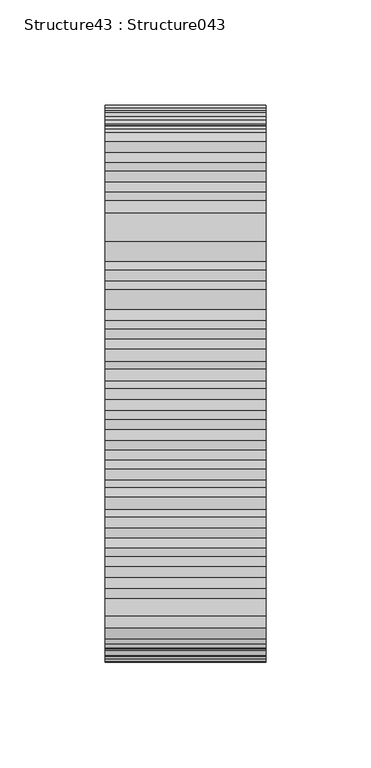
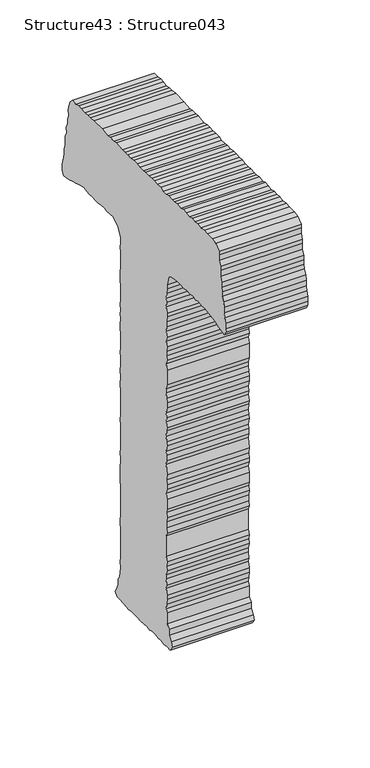
"""IFC4 building model written with IfcOpenShell, lengths in millimetres: proxy geometry, Structure43 : Structure043."""

from ifc_helpers import new_model, si_unit, frame, origin, place, context, project, spatial, polyline, outline, extrude, source, transform, mapped, element, save


def structure43_structure043_932cc00d(model_context):
    return source(origin(), model_context, "Body", "SweptSolid", [
        extrude(outline(polyline([(256415.821603, 3992.8375436), (256417.5818541, 3987.0048063), (256418.7644476, 3982.8793681), (256418.1627209, 3978.2035506), (256419.3437098, 3972.9372387), (256419.922972, 3969.418341), (256421.7056876, 3964.1343784), (256421.103961, 3959.4617701), (256423.4434743, 3954.7506513), (256423.4434743, 3951.2606365), (256423.4434743, 3945.9766739), (256425.2037254, 3940.718385), (256425.2037254, 3937.1930689), (256426.3638545, 3931.3346579), (256427.5448434, 3927.2332888), (256428.7258323, 3923.1319197), (256428.7258323, 3917.8479571), (256425.7845923, 3914.3499193), (256419.922972, 3914.9307861), (256415.2423407, 3916.0909152), (256411.1425762, 3917.8479571), (256406.4619449, 3918.4480792), (256402.9398381, 3919.6066036), (256394.1369778, 3921.9733953), (256388.8786889, 3921.3748778), (256384.7773198, 3920.7908018), (256380.074224, 3921.3748778), (256374.2366728, 3920.7908018), (256370.1353038, 3920.7908018), (256365.432208, 3921.9733953), (256360.173919, 3921.9733953), (256356.6518122, 3921.3748778), (256350.790192, 3921.9733953), (256346.1111652, 3921.9733953), (256337.9100317, 3916.6653636), (256333.7861981, 3909.0627475), (256334.3879248, 3904.3901392), (256334.967187, 3899.1061766), (256334.3879248, 3894.4030808), (256334.3879248, 3885.6210804), (256333.7861981, 3879.7610648), (256334.967187, 3875.0772243), (256334.967187, 3866.8776953), (256333.7861981, 3861.0192843), (256333.7861981, 3857.5019912), (256334.3879248, 3851.6612309), (256333.7861981, 3848.1166595), (256334.967187, 3842.8583706), (256333.7861981, 3837.6000817), (256334.967187, 3834.0474873), (256334.3879248, 3828.2163546), (256334.967187, 3823.5341187), (256334.967187, 3819.4150989), (256334.3879248, 3814.148787), (256334.3879248, 3800.6717138), (256334.967187, 3795.4037973), (256333.7861981, 3791.3056374), (256333.7861981, 3786.0280932), (256334.967187, 3776.6427615), (256333.7861981, 3773.11905), (256334.967187, 3763.759392), (256333.7861981, 3759.0595054), (256333.7861981, 3749.117376), (256334.3879248, 3744.4158848), (256333.7861981, 3738.5574738), (256334.3879248, 3735.0578314), (256334.967187, 3729.7738688), (256333.7861981, 3725.0996559), (256334.3879248, 3720.9726131), (256333.7861981, 3716.2887726), (256333.7861981, 3706.3289925), (256334.3879248, 3702.229228), (256334.967187, 3696.3884676), (256334.3879248, 3692.2710525), (256334.3879248, 3688.1873341), (256334.967187, 3683.4858429), (256334.967187, 3668.8261762), (256333.7861981, 3664.7440624), (256333.7861981, 3655.3587307), (256334.3879248, 3649.5003197), (256334.3879248, 3640.7167147), (256333.7861981, 3636.0408972), (256334.967187, 3631.3410106), (256334.967187, 3627.2396415), (256333.7861981, 3622.555801), (256334.3879248, 3617.2718384), (256334.3879248, 3612.5976255), (256333.7861981, 3607.8961343), (256334.3879248, 3602.6298224), (256334.3879248, 3594.4286888), (256334.967187, 3589.7544759), (256334.3879248, 3583.8864372), (256335.5464492, 3574.5107332), (256337.9100317, 3570.9854171), (256338.4892939, 3565.1254015), (256339.6702828, 3561.6257591), (256342.5890584, 3555.7416744), (256339.6702828, 3552.242032), (256334.967187, 3552.242032), (256330.2881603, 3551.6675836), (256324.4265401, 3551.0658569), (256320.9044332, 3551.0658569), (256316.2254065, 3551.6675836), (256306.843284, 3551.6675836), (256301.5833905, 3551.0658569), (256296.8802947, 3551.6675836), (256291.6204012, 3551.6675836), (256287.5206367, 3551.0658569), (256283.3968031, 3552.242032), (256278.7177764, 3552.242032), (256273.4354184, 3551.6675836), (256269.3565138, 3552.242032), (256264.6774871, 3551.0658569), (256258.7934024, 3552.242032), (256254.1127711, 3551.6675836), (256251.1715311, 3556.3417965), (256252.9317822, 3560.441561), (256255.8746268, 3565.1254015), (256255.8746268, 3570.9854171), (256258.7934024, 3574.5107332), (256259.3726646, 3585.0706354), (256260.5536535, 3588.5702778), (256259.9743913, 3593.2541183), (256259.3726646, 3598.5284533), (256259.3726646, 3602.6298224), (256260.5536535, 3608.4705827), (256259.9743913, 3612.0135494), (256260.5536535, 3617.8559144), (256260.5536535, 3621.9813526), (256259.3726646, 3626.6571701), (256259.9743913, 3630.7392839), (256259.3726646, 3635.4407751), (256260.5536535, 3640.114988), (256260.5536535, 3660.0682449), (256259.3726646, 3663.5598643), (256259.9743913, 3668.2437048), (256259.9743913, 3674.1277895), (256259.3726646, 3678.81163), (256259.9743913, 3683.4858429), (256259.3726646, 3687.0127636), (256259.3726646, 3696.9709391), (256260.5536535, 3702.229228), (256259.3726646, 3706.9130685), (256259.3726646, 3711.0304837), (256259.9743913, 3715.7143242), (256259.3726646, 3720.9726131), (256260.5536535, 3730.3563402), (256259.9743913, 3734.47536), (256259.9743913, 3739.7416719), (256260.5536535, 3743.2332913), (256259.3726646, 3749.701452), (256259.9743913, 3753.2171405), (256260.5536535, 3757.8753073), (256259.9743913, 3763.759392), (256259.3726646, 3767.2590344), (256260.5536535, 3772.5606477), (256259.9743913, 3776.6427615), (256260.5536535, 3781.3282066), (256259.3726646, 3786.6298199), (256259.3726646, 3791.8865042), (256259.9743913, 3795.960595), (256260.5536535, 3800.6717138), (256260.5536535, 3804.7730829), (256259.3726646, 3809.4729695), (256259.3726646, 3823.5341187), (256260.5536535, 3829.374879), (256259.3726646, 3833.4730389), (256259.9743913, 3837.6000817), (256259.9743913, 3842.2758992), (256259.3726646, 3846.9757858), (256260.5536535, 3851.6612309), (256259.3726646, 3856.3161885), (256260.5536535, 3861.6178018), (256259.9743913, 3866.3032469), (256259.9743913, 3870.9790644), (256259.3726646, 3876.263027), (256259.3726646, 3879.7610648), (256260.5536535, 3885.6210804), (256259.9743913, 3890.320967), (256260.5536535, 3893.822214), (256259.9743913, 3899.1061766), (256259.3726646, 3903.7884125), (256259.3726646, 3907.888177), (256257.0556157, 3916.6653636), (256253.5335089, 3919.0321552), (256246.4908997, 3920.7908018), (256240.6308841, 3921.3748778), (256237.1087773, 3921.3748778), (256232.4297505, 3920.7908018), (256227.169857, 3921.3748778), (256222.4667612, 3920.7908018), (256217.2068677, 3921.9733953), (256213.1071032, 3920.7908018), (256209.0057341, 3921.9733953), (256203.1457185, 3920.7908018), (256199.0218849, 3921.3748778), (256185.5608578, 3919.6066036), (256180.8818311, 3918.4480792), (256176.1787353, 3916.6653636), (256172.6790929, 3916.0909152), (256167.3983395, 3914.3499193), (256164.4779594, 3918.4480792), (256165.0572216, 3921.9733953), (256165.0572216, 3927.2332888), (256166.2398151, 3931.9058971), (256167.3983395, 3936.0345445), (256167.3983395, 3941.2912288), (256168.0000662, 3946.5511223), (256170.3171151, 3950.6765605), (256170.9188418, 3954.7506513), (256171.498104, 3958.8776941), (256171.498104, 3963.5615346), (256173.2599598, 3968.2357475), (256173.2599598, 3974.1214368), (256173.2599598, 3978.2035506), (256175.5994731, 3982.8793681), (256175.5994731, 3988.1633307), (256175.5994731, 3991.6806238), (256180.8818311, 3996.390138), (256186.7418467, 3996.9645864), (256194.9429803, 3996.9645864), (256199.6236116, 3997.5486624), (256204.9059696, 3996.9645864), (256210.1658632, 3997.5486624), (256214.8448899, 3996.9645864), (256218.9687234, 3997.5486624), (256223.6477501, 3996.390138), (256228.3283815, 3997.5486624), (256233.6107395, 3997.5486624), (256237.1087773, 3996.390138), (256242.9928619, 3997.5486624), (256247.6734933, 3996.390138), (256251.1715311, 3996.390138), (256256.4538891, 3996.9645864), (256260.5536535, 3996.390138), (256265.2567493, 3996.390138), (256269.9373806, 3997.5486624), (256275.1956696, 3996.9645864), (256279.8987653, 3997.5486624), (256283.9985298, 3997.5486624), (256289.2584234, 3996.9645864), (256294.5407814, 3996.9645864), (256298.0612836, 3996.390138), (256303.9004394, 3996.390138), (256307.4450107, 3997.5486624), (256313.2825619, 3997.5486624), (256317.9856576, 3996.9645864), (256322.666289, 3997.5486624), (256326.7660534, 3997.5486624), (256332.0484114, 3996.390138), (256341.4080695, 3997.5486624), (256345.531903, 3996.9645864), (256350.790192, 3997.5486624), (256354.891561, 3996.390138), (256364.2512191, 3997.5486624), (256377.7571751, 3997.5486624), (256383.6187953, 3996.9645864), (256387.6960954, 3996.9645864), (256392.3991911, 3996.390138), (256397.6590847, 3996.9645864), (256401.7588492, 3997.5486624), (256406.4619449, 3996.390138), (256411.7218385, 3996.9645864), (256415.821603, 3992.8375436)])), frame((-38594.2176606, 0.0, 0.0), z_axis=(1.0, 0.0, 0.0), x_axis=(0.0, 1.0, 0.0)), (0.0, 0.0, 1.0), 76.2),
    ])


if __name__ == "__main__":
    model = new_model("IFC4")
    model_context = context("Model", 3, world=origin())
    ifc_project = project(units=[si_unit("LENGTHUNIT", "METRE", prefix="MILLI")], contexts=[model_context])
    site = spatial("IfcSite", under=ifc_project)
    building = spatial("IfcBuilding", under=site)
    placement = place(None, origin())
    structure43_structure043_shape = structure43_structure043_932cc00d(model_context)
    element("IfcBuildingElementProxy", 1, Name="Structure43 : Structure043", ObjectType="Structure43 : Structure043", at=placement, inside=building, context=model_context, shape_type="MappedRepresentation", body=[
        mapped(structure43_structure043_shape, transform((0.0, 0.0, 0.0), x_axis=(1.0, 0.0, 0.0), y_axis=(0.0, 1.0, 0.0), z_axis=(0.0, 0.0, 1.0))),
    ])
    save(model, "model.ifc")

# Revit data of these elements
# Type "Structure43 : Structure043"
#   NameOverride = "Structure043"
# Element 1 (IfcBuildingElementProxy, "Structure43 : Structure043")
#   Materials on its faces: "BRUSHED ALUM. LETTERING"
# Materials
#   "BRUSHED ALUM. LETTERING": class "Unassigned", colour RGB 169 181 186, transparency 0, Cost = 0
